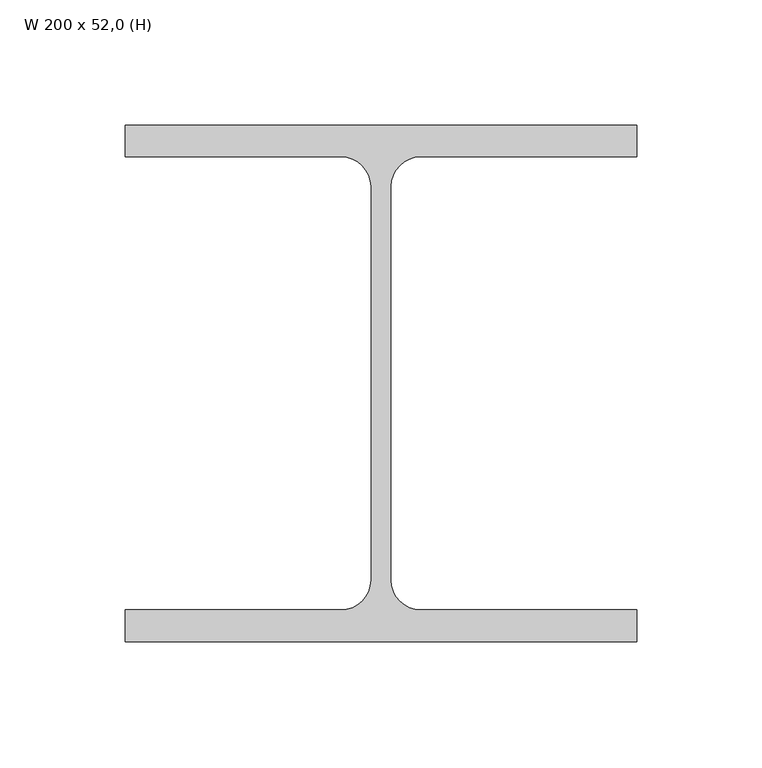
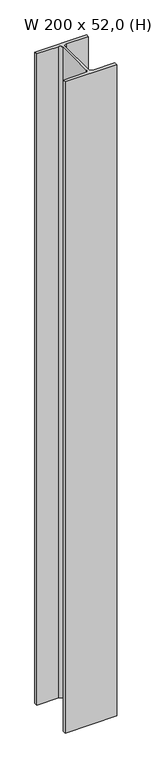
"""IFC4 building model written with IfcOpenShell, lengths in millimetres: column geometry, Pilar de Aço - H : W 200 x 52,0 (H)."""

from ifc_helpers import new_model, si_unit, point, frame_2d, origin, origin_with_axes, place, context, project, spatial, polyline, circle_curve, trimmed, segment, composite_curve, outline, extrude, source, transform, mapped, element, save


def w_200_x_52_0_h_704b740d(model_context):
    return source(origin(), model_context, "Body", "SweptSolid", [
        extrude(outline(composite_curve([segment(polyline([(102.0, 103.0), (102.0, 90.4), (15.85, 90.4)]), True, "CONTINUOUS"), segment(trimmed(circle_curve(frame_2d((15.85, 78.5)), 11.9), [point((15.85, 90.4))], [point((3.95, 78.5))], True, "CARTESIAN"), True, "CONTINUOUS"), segment(polyline([(3.95, 78.5), (3.95, -78.5)]), True, "CONTINUOUS"), segment(trimmed(circle_curve(frame_2d((15.85, -78.5)), 11.9), [point((3.95, -78.5))], [point((15.85, -90.4))], True, "CARTESIAN"), True, "CONTINUOUS"), segment(polyline([(15.85, -90.4), (102.0, -90.4), (102.0, -103.0), (-102.0, -103.0), (-102.0, -90.4), (-15.85, -90.4)]), True, "CONTINUOUS"), segment(trimmed(circle_curve(frame_2d((-15.85, -78.5)), 11.9), [point((-15.85, -90.4))], [point((-3.95, -78.5))], True, "CARTESIAN"), True, "CONTINUOUS"), segment(polyline([(-3.95, -78.5), (-3.95, 78.5)]), True, "CONTINUOUS"), segment(trimmed(circle_curve(frame_2d((-15.85, 78.5)), 11.9), [point((-3.95, 78.5))], [point((-15.85, 90.4))], True, "CARTESIAN"), True, "CONTINUOUS"), segment(polyline([(-15.85, 90.4), (-102.0, 90.4), (-102.0, 103.0), (102.0, 103.0)]), True, "CONTINUOUS")], self_intersect=False)), origin_with_axes(), (0.0, 0.0, 1.0), 2720.0),
    ])


if __name__ == "__main__":
    model = new_model("IFC4")
    model_context = context("Model", 3, world=origin())
    ifc_project = project(units=[si_unit("LENGTHUNIT", "METRE", prefix="MILLI")], contexts=[model_context])
    site = spatial("IfcSite", under=ifc_project)
    building = spatial("IfcBuilding", under=site)
    placement = place(None, origin())
    w_200_x_52_0_h_shape = w_200_x_52_0_h_704b740d(model_context)
    element("IfcColumn", 1, ObjectType="Pilar de Aço - H : W 200 x 52,0 (H)", at=placement, inside=building, context=model_context, shape_type="MappedRepresentation", body=[
        mapped(w_200_x_52_0_h_shape, transform((0.0, 0.0, 0.0), x_axis=(1.0, 0.0, 0.0), y_axis=(0.0, 1.0, 0.0), z_axis=(0.0, 0.0, 1.0))),
    ])
    save(model, "model.ifc")

# Revit data of these elements
# Type "Pilar de Aço - H : W 200 x 52,0 (H)"
#   SINAPI = ""
#   Área da seção = 66.9 m²
#   tw = 0.79 cm
#   tf = 1.26 cm
#   h = 18.08 cm
#   d' = 15.70 cm
#   d = 20.60 cm
#   bf = 20.40 cm
#   R = 1.19 cm
#   Massa Linear kg/m = 52
#   Aço = Metal - Aço 345MPa
#   Assembly Code = ""
# Materials
#   "Metal - Aço 345MPa": class "Metal", colour RGB 189 187 185, transparency 0, Cost = 0
